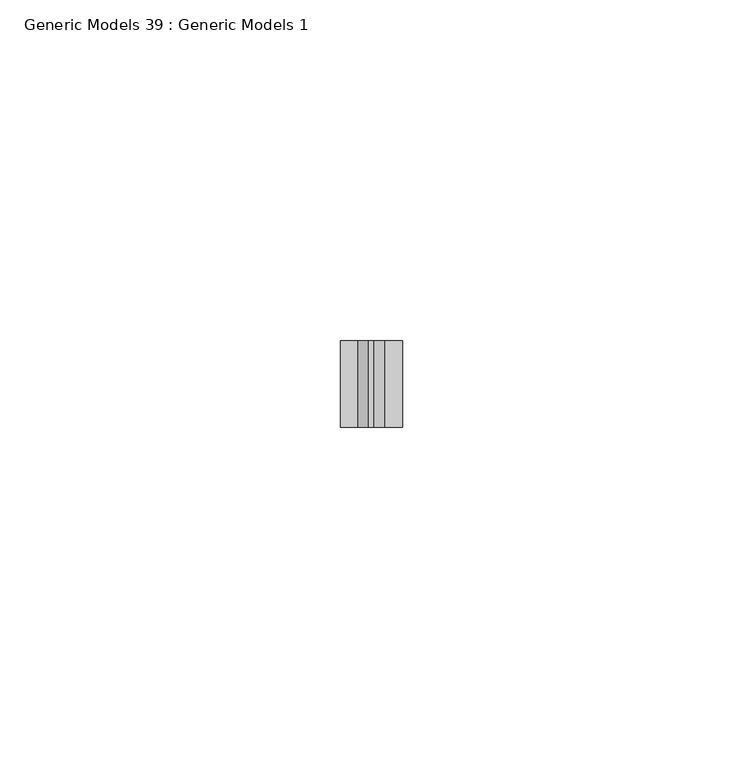
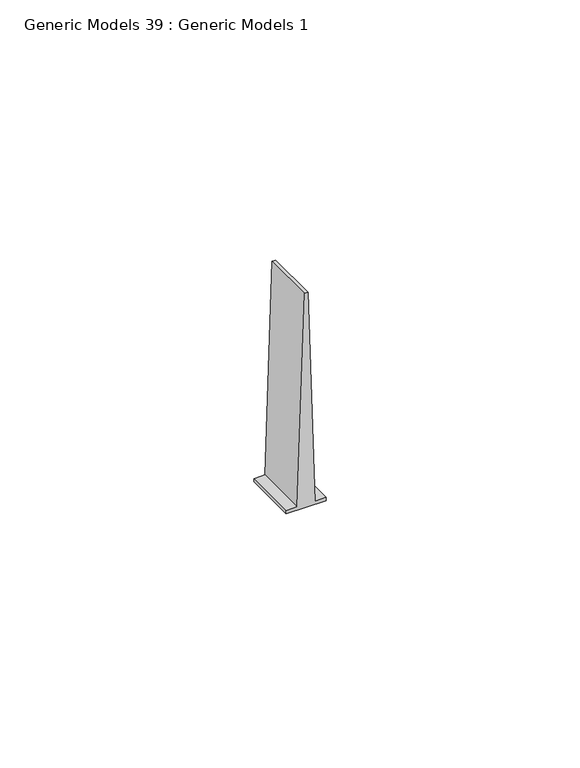
"""IFC4 building model written with IfcOpenShell, lengths in millimetres: proxy geometry, Generic Models 39 : Generic Models 1."""

from ifc_helpers import new_model, si_unit, frame, origin, place, context, project, spatial, polyline, outline, extrude, source, transform, mapped, element, save


def generic_models_39_generic_models_1_7dc37832(model_context):
    return source(origin(), model_context, "Body", "SweptSolid", [
        extrude(outline(polyline([(5263.35625, 49733.4159), (5263.35625, 49742.5091), (5264.15, 49742.5091), (5264.15, 49739.9592364), (5314.95, 49738.3618473), (5314.95, 49737.5631527), (5264.15, 49735.9657636), (5264.15, 49733.4159), (5263.35625, 49733.4159)])), frame((0.0, 565.15, 0.0), z_axis=(0.0, 1.0, 0.0), x_axis=(0.0, 0.0, 1.0)), (0.0, 0.0, 1.0), 12.7),
    ])


if __name__ == "__main__":
    model = new_model("IFC4")
    model_context = context("Model", 3, world=origin())
    ifc_project = project(units=[si_unit("LENGTHUNIT", "METRE", prefix="MILLI")], contexts=[model_context])
    site = spatial("IfcSite", under=ifc_project)
    building = spatial("IfcBuilding", under=site)
    placement = place(None, origin())
    generic_models_39_generic_models_1_shape = generic_models_39_generic_models_1_7dc37832(model_context)
    element("IfcBuildingElementProxy", 1, Name="Generic Models 39 : Generic Models 1", ObjectType="Generic Models 39 : Generic Models 1", at=placement, inside=building, context=model_context, shape_type="MappedRepresentation", body=[
        mapped(generic_models_39_generic_models_1_shape, transform((0.0, 0.0, 0.0), x_axis=(1.0, 0.0, 0.0), y_axis=(0.0, 1.0, 0.0), z_axis=(0.0, 0.0, 1.0))),
    ])
    save(model, "model.ifc")

# Revit data of these elements
# Element 1 (IfcBuildingElementProxy, "Generic Models 39 : Generic Models 1")
#   Materials on its faces: "METAL RUNNER CHANNEL; FASTEN @ 24\" O.C."
# Materials
#   "METAL RUNNER CHANNEL; FASTEN @ 24\" O.C.": class "Unassigned", colour RGB 210 209 208, transparency 0, Keynote = "M05121300.02", Cost = 0
